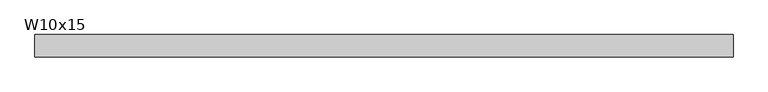
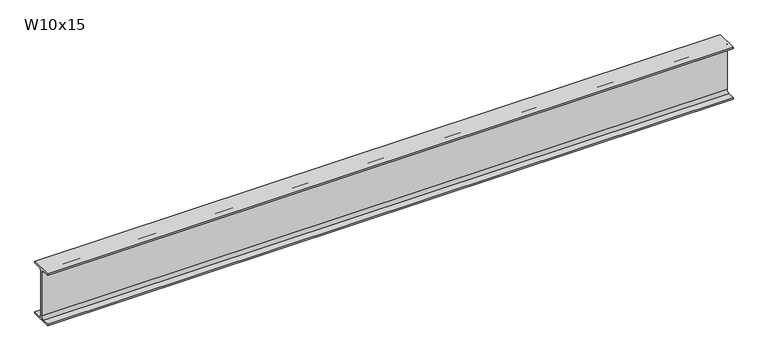
"""IFC4 building model written with IfcOpenShell, lengths in millimetres: beam geometry, RME W-Wide Flange : W10x15."""

from ifc_helpers import new_model, si_unit, point, frame, frame_2d, origin, place, context, project, spatial, polyline, circle_curve, trimmed, segment, composite_curve, outline, extrude, source, transform, mapped, element, save


def w10x15_d71f18f2(model_context):
    return source(origin(), model_context, "Body", "SweptSolid", [
        extrude(outline(composite_curve([segment(polyline([(50.8, -120.142), (50.8, -127.0), (-50.8, -127.0), (-50.8, -120.142), (-16.7005, -120.142)]), True, "CONTINUOUS"), segment(trimmed(circle_curve(frame_2d((-16.7005, -106.3625)), 13.7795), [point((-16.7005, -120.142))], [point((-2.921, -106.3625))], True, "CARTESIAN"), True, "CONTINUOUS"), segment(polyline([(-2.921, -106.3625), (-2.921, 106.3625)]), True, "CONTINUOUS"), segment(trimmed(circle_curve(frame_2d((-16.7005, 106.3625)), 13.7795), [point((-2.921, 106.3625))], [point((-16.7005, 120.142))], True, "CARTESIAN"), True, "CONTINUOUS"), segment(polyline([(-16.7005, 120.142), (-50.8, 120.142), (-50.8, 127.0), (50.8, 127.0), (50.8, 120.142), (16.7005, 120.142)]), True, "CONTINUOUS"), segment(trimmed(circle_curve(frame_2d((16.7005, 106.3625)), 13.7795), [point((16.7005, 120.142))], [point((2.921, 106.3625))], True, "CARTESIAN"), True, "CONTINUOUS"), segment(polyline([(2.921, 106.3625), (2.921, -106.3625)]), True, "CONTINUOUS"), segment(trimmed(circle_curve(frame_2d((16.7005, -106.3625)), 13.7795), [point((2.921, -106.3625))], [point((16.7005, -120.142))], True, "CARTESIAN"), True, "CONTINUOUS"), segment(polyline([(16.7005, -120.142), (50.8, -120.142)]), True, "CONTINUOUS")], self_intersect=False)), frame((-1596.8030222, 0.0, 0.0), z_axis=(1.0, 0.0, 0.0), x_axis=(0.0, 1.0, 0.0)), (0.0, 0.0, 1.0), 3179.8891282),
    ])


if __name__ == "__main__":
    model = new_model("IFC4")
    model_context = context("Model", 3, world=origin())
    ifc_project = project(units=[si_unit("LENGTHUNIT", "METRE", prefix="MILLI")], contexts=[model_context])
    site = spatial("IfcSite", under=ifc_project)
    building = spatial("IfcBuilding", under=site)
    placement = place(None, origin())
    w10x15_shape = w10x15_d71f18f2(model_context)
    element("IfcBeam", 1, ObjectType="RME W-Wide Flange : W10x15", at=placement, inside=building, context=model_context, shape_type="MappedRepresentation", body=[
        mapped(w10x15_shape, transform((0.0, 0.0, 0.0), x_axis=(1.0, 0.0, 0.0), y_axis=(0.0, 1.0, 0.0), z_axis=(0.0, 0.0, 1.0))),
    ])
    save(model, "model.ifc")

# Revit data of these elements
# Type "RME W-Wide Flange : W10x15"
#   WELD P [instance default] = ""
#   WELD LE [instance default] = ""
#   WELD D [instance default] = ""
#   TOP SECTION SIZE [instance default] = ""
#   TOP SECTION LENGTH [instance default] = ""
#   REMARKS [instance default] = ""
#   REINF TYPE [instance default] = ""
#   Nominal Size = "W24"
#   End Bearing Capacity [instance default] = ""
#   BOT SECTION SIZE [instance default] = ""
#   BOT SECTION LENGTH [instance default] = ""
#   Assembly Code = "B10"
#   W = 15
#   Start Extension Calculation [instance default] = 10' - 0"
#   Start Extension [instance default] = -0' - 0 1/2"
#   End Extension Calculation [instance default] = 10' - 0"
#   End Extension [instance default] = -0' - 0 1/2"
#   Length [instance default] = 5' - 0"
#   bf = 0' - 4"
#   d = 0' - 10"
#   k = 0' - 0 13/16"
#   k2 = 0' - 0.5425"
#   tf = 0' - 0.27"
#   tw = 0' - 0.23"
#   A = 0.030625 SF
#   Structural Material [instance default] = Metal - Steel - ASTM A992
# Element 1 (IfcBeam, "RME W-Wide Flange : W10x15")
#   Length = 9' - 11.03177"
#   Materials on its faces: "Metal - Steel - ASTM A992"
# Materials
#   "Metal - Steel - ASTM A992": class "Metal", colour RGB 255 128 0, transparency 0
